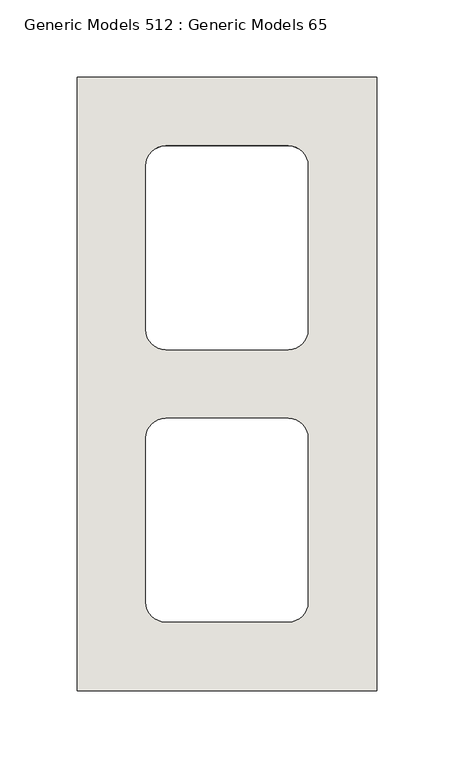
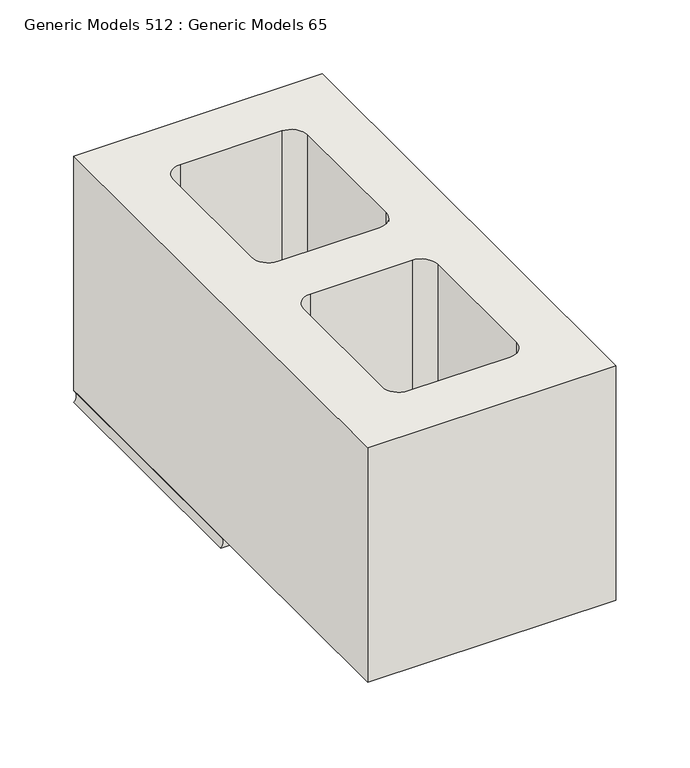
"""IFC4 building model written with IfcOpenShell, lengths in millimetres: wall geometry, Generic Models 512 : Generic Models 65."""

from ifc_helpers import new_model, si_unit, point, frame, frame_2d, origin, place, context, project, spatial, polyline, circle_curve, trimmed, segment, composite_curve, outline, extrude, source, transform, mapped, element, save
from ifc_brep_helpers import plane_surface, revolved_surface, advanced_brep


def generic_models_512_generic_models_65_3aa313c9(model_context):
    return source(origin(), model_context, "Body", "SolidModel", [
        advanced_brep(
        [(428979.0125, 503.2375, 2041.525), (428785.3375, 503.2375, 2041.525), (428785.3375, 503.2375, 2032.0), (428979.0125, 503.2375, 2032.0), (428979.0125, 701.675, 2041.525), (428979.0125, 701.675, 2032.0), (428785.3375, 701.675, 2032.0), (428785.3375, 701.675, 2041.525), (428934.5625, 538.1625, 2041.525), (428921.8625, 525.4625, 2041.525), (428842.4875, 525.4625, 2041.525), (428829.7875, 538.1625, 2041.525), (428829.7875, 644.525, 2041.525), (428842.4875, 657.225, 2041.525), (428921.8625, 657.225, 2041.525), (428934.5625, 644.525, 2041.525), (428921.8625, 525.4625, 2032.0), (428934.5625, 538.1625, 2032.0), (428842.4875, 525.4625, 2032.0), (428829.7875, 538.1625, 2032.0), (428829.7875, 644.525, 2032.0), (428842.4875, 657.225, 2032.0), (428921.8625, 657.225, 2032.0), (428934.5625, 644.525, 2032.0)],
        [
            (0, 1),
            (1, 2, circle_curve(frame((428780.4545028, 503.2375, 2036.7625), z_axis=(0.0, 1.0, 0.0), x_axis=(1.0, 0.0, 0.0)), 6.8209287)),
            (2, 3),
            (3, 0, circle_curve(frame((428983.8954972, 503.2375, 2036.7625), z_axis=(0.0, 1.0, 0.0), x_axis=(-1.0, 0.0, 0.0)), 6.8209287)),
            (4, 5, circle_curve(frame((428983.8954972, 701.675, 2036.7625), z_axis=(0.0, -1.0, 0.0), x_axis=(-1.0, 0.0, 0.0)), 6.8209287)),
            (5, 6),
            (6, 7, circle_curve(frame((428780.4545028, 701.675, 2036.7625), z_axis=(0.0, -1.0, 0.0), x_axis=(1.0, 0.0, 0.0)), 6.8209287)),
            (7, 4),
            (0, 4),
            (7, 1),
            (8, 9, circle_curve(frame((428921.8625, 538.1625, 2041.525), z_axis=(0.0, 0.0, -1.0), x_axis=(-1.0, 0.0, 0.0)), 12.7)),
            (9, 10),
            (10, 11, circle_curve(frame((428842.4875, 538.1625, 2041.525), z_axis=(0.0, 0.0, -1.0), x_axis=(-1.0, 0.0, 0.0)), 12.7)),
            (11, 12),
            (12, 13, circle_curve(frame((428842.4875, 644.525, 2041.525), z_axis=(0.0, 0.0, -1.0), x_axis=(-1.0, 0.0, 0.0)), 12.7)),
            (13, 14),
            (14, 15, circle_curve(frame((428921.8625, 644.525, 2041.525), z_axis=(0.0, 0.0, -1.0), x_axis=(-1.0, 0.0, 0.0)), 12.7)),
            (15, 8),
            (16, 9),
            (8, 17),
            (17, 16, circle_curve(frame((428921.8625, 538.1625, 2032.0), z_axis=(0.0, 0.0, -1.0), x_axis=(-1.0, 0.0, 0.0)), 12.7)),
            (16, 18),
            (18, 10),
            (18, 19, circle_curve(frame((428842.4875, 538.1625, 2032.0), z_axis=(0.0, 0.0, -1.0), x_axis=(-1.0, 0.0, 0.0)), 12.7)),
            (19, 11),
            (19, 20),
            (20, 12),
            (20, 21, circle_curve(frame((428842.4875, 644.525, 2032.0), z_axis=(0.0, 0.0, -1.0), x_axis=(-1.0, 0.0, 0.0)), 12.7)),
            (21, 13),
            (21, 22),
            (22, 14),
            (22, 23, circle_curve(frame((428921.8625, 644.525, 2032.0), z_axis=(0.0, 0.0, -1.0), x_axis=(-1.0, 0.0, 0.0)), 12.7)),
            (23, 15),
            (23, 17),
            (6, 2),
            (5, 3),
        ],
        [
            plane_surface(frame((428882.175, 503.2375, 2041.921875), z_axis=(0.0, -1.0, 0.0), x_axis=(0.0, 0.0, 1.0))),
            plane_surface(frame((428882.175, 701.675, 2041.921875), z_axis=(0.0, 1.0, 0.0), x_axis=(0.0, 0.0, 1.0))),
            plane_surface(frame((428979.0125, 503.2375, 2041.525), z_axis=(0.0, 0.0, 1.0), x_axis=(0.0, 1.0, 0.0))),
            revolved_surface(polyline([(428909.1625, 538.1625, 2041.525), (428909.1625, 538.1625, 2032.0)]), (428921.8625, 538.1625, 2225.675), (0.0, 0.0, 1.0)),
            plane_surface(frame((428842.4875, 525.4625, 2225.675), z_axis=(0.0, 1.0, 0.0), x_axis=(0.0, 0.0, -1.0))),
            revolved_surface(polyline([(428829.7875, 538.1625, 2041.525), (428829.7875, 538.1625, 2032.0)]), (428842.4875, 538.1625, 2225.675), (0.0, 0.0, 1.0)),
            plane_surface(frame((428829.7875, 644.525, 2225.675), z_axis=(1.0, 0.0, 0.0), x_axis=(0.0, 0.0, -1.0))),
            revolved_surface(polyline([(428829.7875, 644.525, 2041.525), (428829.7875, 644.525, 2032.0)]), (428842.4875, 644.525, 2225.675), (0.0, 0.0, 1.0)),
            plane_surface(frame((428921.8625, 657.225, 2225.675), z_axis=(0.0, -1.0, 0.0), x_axis=(0.0, 0.0, -1.0))),
            revolved_surface(polyline([(428909.1625, 644.525, 2041.525), (428909.1625, 644.525, 2032.0)]), (428921.8625, 644.525, 2225.675), (0.0, 0.0, 1.0)),
            plane_surface(frame((428934.5625, 538.1625, 2225.675), z_axis=(-1.0, 0.0, 0.0), x_axis=(0.0, 0.0, -1.0))),
            revolved_surface(polyline([(428787.2754315, 701.675, 2036.7625), (428787.2754315, 503.2375, 2036.7625)]), (428780.4545028, 503.2375, 2036.7625), (0.0, 1.0, 0.0)),
            plane_surface(frame((428785.3375, 503.2375, 2032.0), z_axis=(0.0, 0.0, -1.0), x_axis=(0.0, 1.0, 0.0))),
            revolved_surface(polyline([(428977.07456850004, 701.675, 2036.7625), (428977.07456850004, 503.2375, 2036.7625)]), (428983.8954972, 503.2375, 2036.7625), (0.0, 1.0, 0.0)),
        ],
        [
            (0, [[1, 2, 3, 4]]),
            (1, [[5, 6, 7, 8]]),
            (2, [[-1, 9, -8, 10], [11, 12, 13, 14, 15, 16, 17, 18]]),
            (3, [[19, -11, 20, 21]]),
            (4, [[-19, 22, 23, -12]]),
            (5, [[-23, 24, 25, -13]]),
            (6, [[-25, 26, 27, -14]]),
            (7, [[-27, 28, 29, -15]]),
            (8, [[-29, 30, 31, -16]]),
            (9, [[-31, 32, 33, -17]]),
            (10, [[-33, 34, -20, -18]]),
            (11, [[-2, -10, -7, 35]]),
            (12, [[-3, -35, -6, 36], [-21, -34, -32, -30, -28, -26, -24, -22]]),
            (13, [[-4, -36, -5, -9]]),
        ],
    ),
        extrude(outline(polyline([(428979.0125, 304.8), (428785.3375, 304.8), (428785.3375, 701.675), (428979.0125, 701.675), (428979.0125, 304.8)]), holes=[composite_curve([segment(polyline([(428934.5625, 538.1625), (428934.5625, 644.525)]), True, "CONTINUOUS"), segment(trimmed(circle_curve(frame_2d((428921.8625, 644.525)), 12.7), [point((428934.5625, 644.525))], [point((428921.8625, 657.225))], True, "CARTESIAN"), True, "CONTINUOUS"), segment(polyline([(428921.8625, 657.225), (428842.4875, 657.225)]), True, "CONTINUOUS"), segment(trimmed(circle_curve(frame_2d((428842.4875, 644.525)), 12.7), [point((428842.4875, 657.225))], [point((428829.7875, 644.525))], True, "CARTESIAN"), True, "CONTINUOUS"), segment(polyline([(428829.7875, 644.525), (428829.7875, 538.1625)]), True, "CONTINUOUS"), segment(trimmed(circle_curve(frame_2d((428842.4875, 538.1625)), 12.7), [point((428829.7875, 538.1625))], [point((428842.4875, 525.4625))], True, "CARTESIAN"), True, "CONTINUOUS"), segment(polyline([(428842.4875, 525.4625), (428921.8625, 525.4625)]), True, "CONTINUOUS"), segment(trimmed(circle_curve(frame_2d((428921.8625, 538.1625)), 12.7), [point((428921.8625, 525.4625))], [point((428934.5625, 538.1625))], True, "CARTESIAN"), True, "CONTINUOUS")], self_intersect=False), composite_curve([segment(polyline([(428829.7875, 468.3125), (428829.7875, 361.95)]), True, "CONTINUOUS"), segment(trimmed(circle_curve(frame_2d((428842.4875, 361.95)), 12.7), [point((428829.7875, 361.95))], [point((428842.4875, 349.25))], True, "CARTESIAN"), True, "CONTINUOUS"), segment(polyline([(428842.4875, 349.25), (428921.8625, 349.25)]), True, "CONTINUOUS"), segment(trimmed(circle_curve(frame_2d((428921.8625, 361.95)), 12.7), [point((428921.8625, 349.25))], [point((428934.5625, 361.95))], True, "CARTESIAN"), True, "CONTINUOUS"), segment(polyline([(428934.5625, 361.95), (428934.5625, 468.3125)]), True, "CONTINUOUS"), segment(trimmed(circle_curve(frame_2d((428921.8625, 468.3125)), 12.7), [point((428934.5625, 468.3125))], [point((428921.8625, 481.0125))], True, "CARTESIAN"), True, "CONTINUOUS"), segment(polyline([(428921.8625, 481.0125), (428842.4875, 481.0125)]), True, "CONTINUOUS"), segment(trimmed(circle_curve(frame_2d((428842.4875, 468.3125)), 12.7), [point((428842.4875, 481.0125))], [point((428829.7875, 468.3125))], True, "CARTESIAN"), True, "CONTINUOUS")], self_intersect=False)]), frame((0.0, 0.0, 2041.525), z_axis=(0.0, 0.0, 1.0), x_axis=(1.0, 0.0, 0.0)), (0.0, 0.0, 1.0), 193.675),
    ])


if __name__ == "__main__":
    model = new_model("IFC4")
    model_context = context("Model", 3, world=origin())
    ifc_project = project(units=[si_unit("LENGTHUNIT", "METRE", prefix="MILLI")], contexts=[model_context])
    site = spatial("IfcSite", under=ifc_project)
    building = spatial("IfcBuilding", under=site)
    placement = place(None, origin())
    generic_models_512_generic_models_65_shape = generic_models_512_generic_models_65_3aa313c9(model_context)
    element("IfcWall", 1, ObjectType="Generic Models 512 : Generic Models 65", at=placement, inside=building, context=model_context, shape_type="MappedRepresentation", body=[
        mapped(generic_models_512_generic_models_65_shape, transform((0.0, 0.0, 0.0), x_axis=(1.0, 0.0, 0.0), y_axis=(0.0, 1.0, 0.0), z_axis=(0.0, 0.0, 1.0))),
    ])
    save(model, "model.ifc")

# Revit data of these elements
# Element 1 (IfcWall, "Generic Models 512 : Generic Models 65")
#   Materials on its faces: "CMU (SEE 'WALL TAG' FOR SIZE)", "MORTAR JOINT"
# Materials
#   "CMU (SEE 'WALL TAG' FOR SIZE)": class "Masonry", colour RGB 203 203 199, transparency 0, Description = "Concrete masonry units", Cost = 0
#   "MORTAR JOINT": class "Generic", colour RGB 120 120 120, transparency 0, Cost = 0
